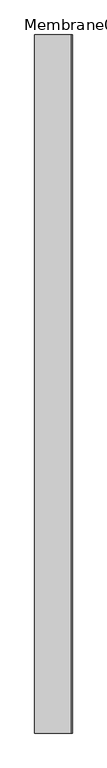
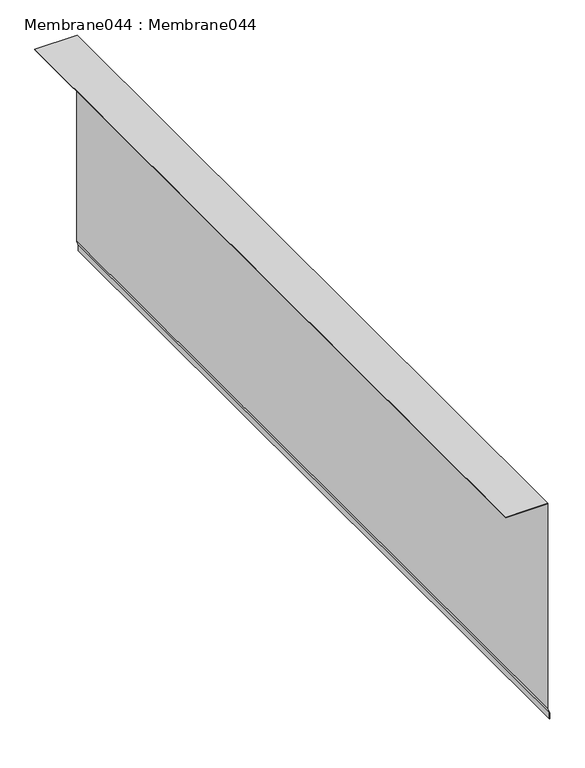
"""IFC4 building model written with IfcOpenShell, lengths in millimetres: proxy geometry, Membrane044 : Membrane044."""

from ifc_helpers import new_model, si_unit, frame, origin, place, context, project, spatial, polyline, outline, extrude, source, transform, mapped, element, save


def membrane044_membrane044_564da0ca(model_context):
    return source(origin(), model_context, "Body", "SweptSolid", [
        extrude(outline(polyline([(40112.683796, -9398.2396626), (40111.683796, -9398.2396626), (40111.683796, -9295.4978798), (39579.3230707, -9295.4978798), (39568.0978055, -9291.4122174), (39552.6918208, -9291.4122174), (39552.6918208, -9290.4122174), (39568.2741325, -9290.4122174), (39579.4993977, -9294.4978798), (40112.683796, -9294.4978798), (40112.683796, -9398.2396626)])), frame((0.0, 7182.1531721, 0.0), z_axis=(0.0, 1.0, 0.0), x_axis=(0.0, 0.0, 1.0)), (0.0, 0.0, 1.0), 2000.0),
    ])


if __name__ == "__main__":
    model = new_model("IFC4")
    model_context = context("Model", 3, world=origin())
    ifc_project = project(units=[si_unit("LENGTHUNIT", "METRE", prefix="MILLI")], contexts=[model_context])
    site = spatial("IfcSite", under=ifc_project)
    building = spatial("IfcBuilding", under=site)
    placement = place(None, origin())
    membrane044_membrane044_shape = membrane044_membrane044_564da0ca(model_context)
    element("IfcBuildingElementProxy", 1, Name="Membrane044 : Membrane044", ObjectType="Membrane044 : Membrane044", at=placement, inside=building, context=model_context, shape_type="MappedRepresentation", body=[
        mapped(membrane044_membrane044_shape, transform((0.0, 0.0, 0.0), x_axis=(1.0, 0.0, 0.0), y_axis=(0.0, 1.0, 0.0), z_axis=(0.0, 0.0, 1.0))),
    ])
    save(model, "model.ifc")

# Revit data of these elements
# Type "Membrane044 : Membrane044"
#   NameOverride = "Membrane044"
# Element 1 (IfcBuildingElementProxy, "Membrane044 : Membrane044")
#   Materials on its faces: "(2) LAYERS OF ICE & WATER SHIELD (BITUTHANE) UNDER STUCCO"
# Materials
#   "(2) LAYERS OF ICE & WATER SHIELD (BITUTHANE) UNDER STUCCO": class "Unassigned", colour RGB 186 255 159, transparency 0, Cost = 0
